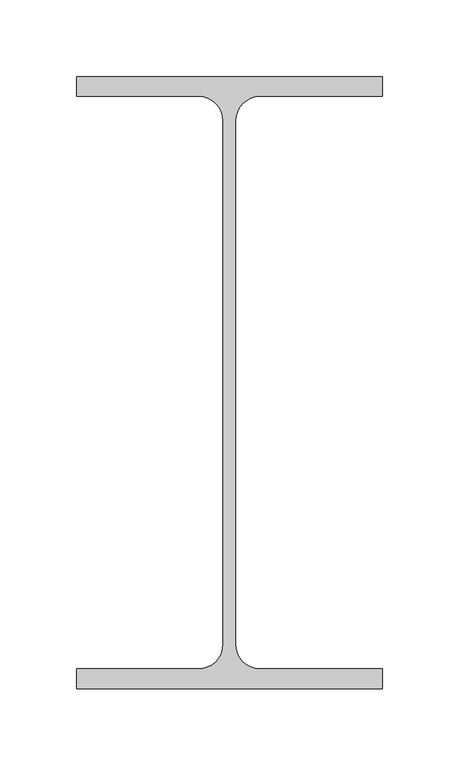
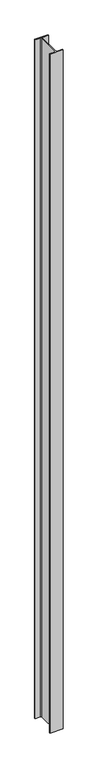
"""IFC4 building model written with IfcOpenShell, lengths in millimetres: column geometry, 0912_Steel Column_H_KSD3502 : H_SC_ASC_H-400x200x8x13."""

from ifc_helpers import new_model, si_unit, point, frame, frame_2d, origin, place, context, project, spatial, polyline, circle_curve, trimmed, segment, composite_curve, outline, extrude, source, transform, mapped, element, save


def column_8add4d16(model_context):
    return source(origin(), model_context, "Body", "SweptSolid", [
        extrude(outline(composite_curve([segment(polyline([(100.0, 200.0), (100.0, 187.0), (20.0, 187.0)]), True, "CONTINUOUS"), segment(trimmed(circle_curve(frame_2d((20.0, 171.0)), 16.0), [point((20.0, 187.0))], [point((4.0, 171.0))], True, "CARTESIAN"), True, "CONTINUOUS"), segment(polyline([(4.0, 171.0), (4.0, -171.0)]), True, "CONTINUOUS"), segment(trimmed(circle_curve(frame_2d((20.0, -171.0)), 16.0), [point((4.0, -171.0))], [point((20.0, -187.0))], True, "CARTESIAN"), True, "CONTINUOUS"), segment(polyline([(20.0, -187.0), (100.0, -187.0), (100.0, -200.0), (-100.0, -200.0), (-100.0, -187.0), (-20.0, -187.0)]), True, "CONTINUOUS"), segment(trimmed(circle_curve(frame_2d((-20.0, -171.0)), 16.0), [point((-20.0, -187.0))], [point((-4.0, -171.0))], True, "CARTESIAN"), True, "CONTINUOUS"), segment(polyline([(-4.0, -171.0), (-4.0, 171.0)]), True, "CONTINUOUS"), segment(trimmed(circle_curve(frame_2d((-20.0, 171.0)), 16.0), [point((-4.0, 171.0))], [point((-20.0, 187.0))], True, "CARTESIAN"), True, "CONTINUOUS"), segment(polyline([(-20.0, 187.0), (-100.0, 187.0), (-100.0, 200.0), (100.0, 200.0)]), True, "CONTINUOUS")], self_intersect=False)), frame((0.0, 0.0, 7249.9720055), z_axis=(0.0, 0.0, 1.0), x_axis=(1.0, 0.0, 0.0)), (0.0, 0.0, 1.0), 10950.0),
    ])


if __name__ == "__main__":
    model = new_model("IFC4")
    model_context = context("Model", 3, world=origin())
    ifc_project = project(units=[si_unit("LENGTHUNIT", "METRE", prefix="MILLI")], contexts=[model_context])
    site = spatial("IfcSite", under=ifc_project)
    building = spatial("IfcBuilding", under=site)
    placement = place(None, origin())
    column_shape = column_8add4d16(model_context)
    element("IfcColumn", 1, ObjectType="0912_Steel Column_H_KSD3502 : H_SC_ASC_H-400x200x8x13", at=placement, inside=building, context=model_context, shape_type="MappedRepresentation", body=[
        mapped(column_shape, transform((0.0, 0.0, 0.0), x_axis=(1.0, 0.0, 0.0), y_axis=(0.0, 1.0, 0.0), z_axis=(0.0, 0.0, 1.0))),
    ])
    save(model, "model.ifc")

# Revit data of these elements
# Type "0912_Steel Column_H_KSD3502 : H_SC_ASC_H-400x200x8x13"
#   H_WM Code_1 = "S01AA002-00001 | Main Steel Structure Fabrication Work | Shelter/Building | Medium Steel - Standard (90KG/M>Weight≥30KG/M) | Material: (   )"
#   H_WM Code_2 = "S03AA028-00001 | Main Steel Structure Erection Work | Shelter/Building | Medium Steel (90KG/M>Weight≥30KG/M) | Material: (   )"
#   H_WM Code_3 = "S01AA010-00001 | Main Steel Structure Fabrication Work | Shelter/Building | Steel Painting/Coating | for Non-Fireproofed Steel Surface, Surface Preparation, Primer, Second & Final Coat | Material: (   )"
#   H_Q'ty Cal Type Tag = "SC-Q2"
#   Width = 20.0 cm
#   Web Thickness = 0.8 cm
#   Web Fillet = 1.6 cm
#   Warping Constant = 648999.0 cm⁶
#   Torsional Moment of Inertia = 35.8981 cm⁴
#   Section Area = 84.12 cm²
#   Plastic Modulus weak axis = 268.0 cm³
#   Plastic Modulus strong axis = 1330.0 cm³
#   Perimeter = 1.56 m²/m
#   Nominal Weight = 66.00 kgf/m
#   Moment of Inertia weak axis = 1740.00 cm⁴
#   Moment of Inertia strong axis = 23700.00 cm⁴
#   Height = 40.0 cm
#   Flange Thickness = 1.3 cm
#   Elastic Modulus weak axis = 174.0 cm³
#   Elastic Modulus strong axis = 1190.0 cm³
#   Centroid Vertical = 20.0 cm
#   Centroid Horizontal = 10.0 cm
#   Structural Material [instance default] = Steel, 45-345
#   Section Name Key = ""
#   Bolt Spacing = 0
#   Assembly Code = ""
# Element 1 (IfcColumn, "0912_Steel Column_H_KSD3502 : H_SC_ASC_H-400x200x8x13")
#   Structural Material = none
# Materials
#   "Steel, 45-345": class "Metal", colour RGB 189 187 185, transparency 0, Description = "Steel 345 MPa", Cost = 0
